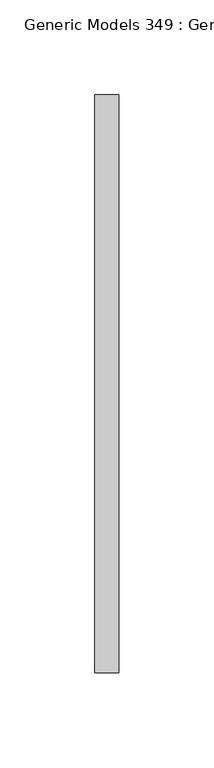
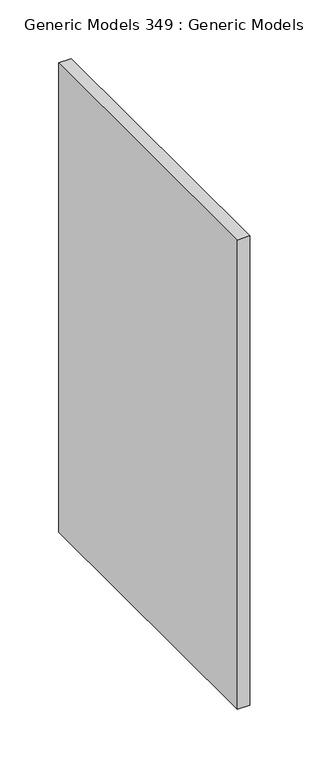
"""IFC4 building model written with IfcOpenShell, lengths in millimetres: proxy geometry, Generic Models 349 : Generic Models 349."""

from ifc_helpers import new_model, si_unit, frame, origin, place, context, project, spatial, polyline, outline, extrude, source, transform, mapped, element, save


def generic_models_349_generic_models_349_82dd0115(model_context):
    return source(origin(), model_context, "Body", "SweptSolid", [
        extrude(outline(polyline([(-6439.0736296, -4250.542257), (-6451.7736295, -4250.542257), (-6451.7736295, -3945.742257), (-6439.0736296, -3945.742257), (-6439.0736296, -4250.542257)])), frame((0.0, 0.0, 126783.846), z_axis=(0.0, 0.0, 1.0), x_axis=(1.0, 0.0, 0.0)), (0.0, 0.0, 1.0), 488.95),
    ])


if __name__ == "__main__":
    model = new_model("IFC4")
    model_context = context("Model", 3, world=origin())
    ifc_project = project(units=[si_unit("LENGTHUNIT", "METRE", prefix="MILLI")], contexts=[model_context])
    site = spatial("IfcSite", under=ifc_project)
    building = spatial("IfcBuilding", under=site)
    placement = place(None, origin())
    generic_models_349_generic_models_349_shape = generic_models_349_generic_models_349_82dd0115(model_context)
    element("IfcBuildingElementProxy", 1, Name="Generic Models 349 : Generic Models 349", ObjectType="Generic Models 349 : Generic Models 349", at=placement, inside=building, context=model_context, shape_type="MappedRepresentation", body=[
        mapped(generic_models_349_generic_models_349_shape, transform((0.0, 0.0, 0.0), x_axis=(1.0, 0.0, 0.0), y_axis=(0.0, 1.0, 0.0), z_axis=(0.0, 0.0, 1.0))),
    ])
    save(model, "model.ifc")

# Revit data of these elements
# Element 1 (IfcBuildingElementProxy, "Generic Models 349 : Generic Models 349")
#   Materials on its faces: "_5/8\" DRYWALL"
# Materials
#   "_5/8\" DRYWALL": class "Generic", colour RGB 191 191 191, transparency 0, Cost = 0
